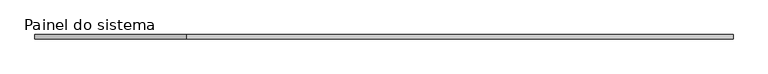
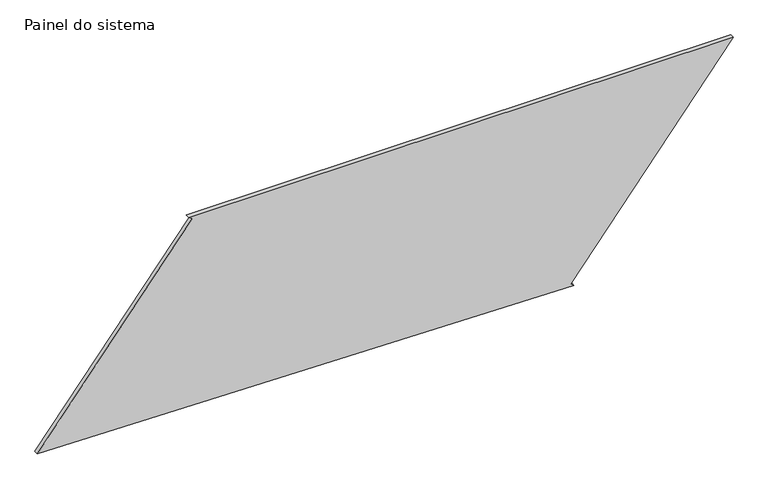
"""IFC4 building model written with IfcOpenShell, lengths in millimetres: plate geometry, Painel do sistema : Envidraçado."""

import ifcopenshell
import ifcopenshell.guid

model = None  # the IFC model being written
_history = None  # IfcOwnerHistory: only IFC2X3 demands one
_inside = {}  # id of a spatial element -> (the spatial element, [elements in it])
_under = {}  # id of a project, library or spatial element -> (it, [spatial elements below it])
_declared = {}  # id of a project -> (the project, [libraries it declares])
_typed = {}  # id of a type object -> (the type object, [elements of that type])
_made_of = {}  # id of a material, layer set ... -> (it, [elements and type objects made of it])


def new_model(schema):
    """Start an empty IFC model of exactly this schema.

    Asked for "IFC4X3", IfcOpenShell would pick the latest addendum, in which some entities
    have other attributes; the version numbers below select the first issue.
    IFC2X3 requires an IfcOwnerHistory on every rooted entity: one is made here for all.
    """
    global model, _history
    if schema == "IFC4X3":
        model = ifcopenshell.file(schema_version=(4, 3, 0, 0))
    else:
        model = ifcopenshell.file(schema=schema)
    _inside.clear()
    _under.clear()
    _declared.clear()
    _typed.clear()
    _made_of.clear()
    _history = None
    if model.schema == "IFC2X3":
        org = make("IfcOrganization", Name="unknown")
        user = make(
            "IfcPersonAndOrganization",
            ThePerson=make("IfcPerson", FamilyName="unknown"),
            TheOrganization=org,
        )
        app = make(
            "IfcApplication",
            ApplicationDeveloper=org,
            Version="unknown",
            ApplicationFullName="unknown",
            ApplicationIdentifier="unknown",
        )
        _history = make(
            "IfcOwnerHistory",
            OwningUser=user,
            OwningApplication=app,
            ChangeAction="ADDED",
            CreationDate=0,
        )
    return model


def make(cls, **values):
    """One entity of the class cls with the attributes given. An attribute that is None is left unset."""
    return model.create_entity(
        cls, **{name: value for name, value in values.items() if value is not None}
    )


def rooted(cls, **values):
    """An entity with a GlobalId (a new one), such as an element, a storey or a relation."""
    return make(cls, GlobalId=ifcopenshell.guid.new(), OwnerHistory=_history, **values)


def si_unit(unit_type, name, prefix=None):
    """IfcSIUnit, for example si_unit("LENGTHUNIT", "METRE", prefix="MILLI")."""
    return make("IfcSIUnit", UnitType=unit_type, Prefix=prefix, Name=name)


def assignment(units):
    """IfcUnitAssignment: the units of a project."""
    return None if units is None else make("IfcUnitAssignment", Units=units)


def point(xyz):
    """IfcCartesianPoint."""
    return None if xyz is None else make("IfcCartesianPoint", Coordinates=xyz)


def direction(xyz):
    """IfcDirection."""
    return None if xyz is None else make("IfcDirection", DirectionRatios=xyz)


def frame(location, z_axis=None, x_axis=None):
    """IfcAxis2Placement3D, a coordinate frame: its origin and axes. An axis left out is left unset."""
    return make(
        "IfcAxis2Placement3D",
        Location=point(location),
        Axis=direction(z_axis),
        RefDirection=direction(x_axis),
    )


def origin():
    """The frame at (0, 0, 0) with its axes left unset."""
    return frame((0.0, 0.0, 0.0))


def place(relative_to, where):
    """IfcLocalPlacement: puts the frame where relative to a parent placement (None: the world)."""
    return make(
        "IfcLocalPlacement", PlacementRelTo=relative_to, RelativePlacement=where
    )


def context(
    kind, dimensions, precision=None, world=None, true_north=None, identifier=None
):
    """IfcGeometricRepresentationContext, for example the 3D "Model" context."""
    return make(
        "IfcGeometricRepresentationContext",
        ContextIdentifier=identifier,
        ContextType=kind,
        CoordinateSpaceDimension=dimensions,
        Precision=precision,
        WorldCoordinateSystem=world,
        TrueNorth=true_north,
    )


def project(units=None, contexts=None):
    """IfcProject with its units and contexts."""
    return rooted(
        "IfcProject",
        Name="project",
        RepresentationContexts=contexts,
        UnitsInContext=assignment(units),
    )


def spatial(cls, under=None, at=None, **own):
    """A site, building, storey or space (cls), placed at a placement, below another one or the project."""
    s = rooted(cls, ObjectPlacement=at, **own)
    if under is not None:
        _under.setdefault(under.id(), (under, []))[1].append(s)
    return s


def polyline(points):
    """IfcPolyline through the points."""
    return make("IfcPolyline", Points=[point(p) for p in points])


def outline(outer, holes=None, kind="AREA"):
    """IfcArbitraryClosedProfileDef: a profile drawn as a closed curve; with holes, ...WithVoids."""
    if holes is None:
        return make("IfcArbitraryClosedProfileDef", ProfileType=kind, OuterCurve=outer)
    return make(
        "IfcArbitraryProfileDefWithVoids",
        ProfileType=kind,
        OuterCurve=outer,
        InnerCurves=holes,
    )


def extrude(swept, where, along, depth):
    """IfcExtrudedAreaSolid: the profile swept, set in the frame where, extruded along a direction by depth."""
    return make(
        "IfcExtrudedAreaSolid",
        SweptArea=swept,
        Position=where,
        ExtrudedDirection=direction(along),
        Depth=depth,
    )


def shape(context_of_items, identifier, shape_type, items):
    """IfcShapeRepresentation: the items that make up one representation, for example the "Body"."""
    return make(
        "IfcShapeRepresentation",
        ContextOfItems=context_of_items,
        RepresentationIdentifier=identifier,
        RepresentationType=shape_type,
        Items=items,
    )


def source(mapping_origin, context_of_items, identifier, shape_type, items):
    """IfcRepresentationMap: a shape defined once, which mapped items show again and again."""
    return make(
        "IfcRepresentationMap",
        MappingOrigin=mapping_origin,
        MappedRepresentation=shape(context_of_items, identifier, shape_type, items),
    )


def transform(
    local_origin,
    x_axis=None,
    y_axis=None,
    z_axis=None,
    scale=None,
    scale2=None,
    scale3=None,
    uniform=True,
):
    """IfcCartesianTransformationOperator3D, or its non-uniform kind. x_axis, y_axis, z_axis: its Axis1, 2, 3."""
    if uniform:
        return make(
            "IfcCartesianTransformationOperator3D",
            Axis1=direction(x_axis),
            Axis2=direction(y_axis),
            LocalOrigin=point(local_origin),
            Scale=scale,
            Axis3=direction(z_axis),
        )
    return make(
        "IfcCartesianTransformationOperator3DnonUniform",
        Axis1=direction(x_axis),
        Axis2=direction(y_axis),
        LocalOrigin=point(local_origin),
        Scale=scale,
        Axis3=direction(z_axis),
        Scale2=scale2,
        Scale3=scale3,
    )


def mapped(mapping_source, mapping_target):
    """IfcMappedItem: shows the shape of a source again, moved by a transform."""
    return make(
        "IfcMappedItem", MappingSource=mapping_source, MappingTarget=mapping_target
    )


def made_of(thing, what):
    """Note that an element or type object is made of a material, layer set ...; save() writes the relation."""
    if what is not None:
        _made_of.setdefault(what.id(), (what, []))[1].append(thing)
    return thing


def element(
    cls,
    number,
    at=None,
    inside=None,
    cuts=None,
    type_object=None,
    material=None,
    context=None,
    identifier="Body",
    shape_type=None,
    held_by="IfcProductDefinitionShape",
    body=None,
    shapes=None,
    **own,
):
    """One element of the class cls, such as IfcWall. Its Tag is "e" and its number.

    at: its placement. inside: the storey or other place that contains it. cuts: it is an
    opening in that element (IfcRelVoidsElement). A single representation is given by context,
    identifier, shape_type and body (its items); several are given by shapes. held_by: the class
    of the entity that holds the representations. save() writes the other relations.
    """
    e = rooted(cls, Tag="e%d" % number, ObjectPlacement=at, **own)
    if body is not None:
        shapes = [shape(context, identifier, shape_type, body)]
    if shapes is not None:
        e.Representation = make(held_by, Representations=shapes)
    if inside is not None:
        _inside.setdefault(inside.id(), (inside, []))[1].append(e)
    if cuts is not None:
        rooted(
            "IfcRelVoidsElement", RelatingBuildingElement=cuts, RelatedOpeningElement=e
        )
    if type_object is not None:
        _typed.setdefault(type_object.id(), (type_object, []))[1].append(e)
    return made_of(e, material)


def aggregate(whole, parts):
    """IfcRelAggregates: a whole, such as a stair, and the parts it consists of."""
    return rooted("IfcRelAggregates", RelatingObject=whole, RelatedObjects=parts)


def save(model, path):
    """Write the relations noted so far, then the file.

    IfcRelAggregates (storeys below a building ...), IfcRelContainedInSpatialStructure (elements
    in a storey), IfcRelDefinesByType, IfcRelAssociatesMaterial and IfcRelDeclares: one each for
    every whole, place, type object, material and project.
    """
    for whole, parts in _under.values():
        aggregate(whole, parts)
    for where, things in _inside.values():
        rooted(
            "IfcRelContainedInSpatialStructure",
            RelatedElements=things,
            RelatingStructure=where,
        )
    for kind, things in _typed.values():
        rooted("IfcRelDefinesByType", RelatedObjects=things, RelatingType=kind)
    for what, things in _made_of.values():
        rooted("IfcRelAssociatesMaterial", RelatedObjects=things, RelatingMaterial=what)
    for by, libraries in _declared.values():
        rooted("IfcRelDeclares", RelatingContext=by, RelatedDefinitions=libraries)
    model.write(path)


def painel_do_sistema_68b5d6e9(model_context):
    return source(origin(), model_context, "Body", "SweptSolid", [
        extrude(outline(polyline([(0.0, 1128.6359159), (15.5601026, 1109.0685143), (1237.1544126, 2080.4868549), (1237.1544126, -1174.4534105), (1221.59431, -1154.8860089), (57.6171855, -2080.4868549), (0.0, 1128.6359159)])), frame((0.0, 24.5, 0.0), z_axis=(0.0, 1.0, 0.0), x_axis=(0.0, 0.0, 1.0)), (0.0, 0.0, 1.0), 25.0),
    ])


if __name__ == "__main__":
    model = new_model("IFC4")
    model_context = context("Model", 3, world=origin())
    ifc_project = project(units=[si_unit("LENGTHUNIT", "METRE", prefix="MILLI")], contexts=[model_context])
    site = spatial("IfcSite", under=ifc_project)
    building = spatial("IfcBuilding", under=site)
    placement = place(None, origin())
    painel_do_sistema_shape = painel_do_sistema_68b5d6e9(model_context)
    element("IfcPlate", 1, ObjectType="Painel do sistema : Envidraçado", at=placement, inside=building, context=model_context, shape_type="MappedRepresentation", body=[
        mapped(painel_do_sistema_shape, transform((0.0, 0.0, 0.0), x_axis=(1.0, 0.0, 0.0), y_axis=(0.0, 1.0, 0.0), z_axis=(0.0, 0.0, 1.0))),
    ])
    save(model, "model.ifc")

# Revit data of these elements
# Type "Painel do sistema : Envidraçado"
#   Construction Type Id = "GSP4R"
#   Analytic Construction = "Vidraça única Pilkington 1/8 pol"
#   Visual Light Transmittance = 0.9
#   Solar Heat Gain Coefficient = 0.86
#   Heat Transfer Coefficient (U) = 6.7069 W/(m²·K)
# Element 1 (IfcPlate, "Painel do sistema : Envidraçado")
#   Materials on its faces: "Vidro"
# Materials
#   "Vidro": class "Vidro", colour RGB 0 128 192, transparency 0.9, Description = "Vidro de sílica", Cost = 0
